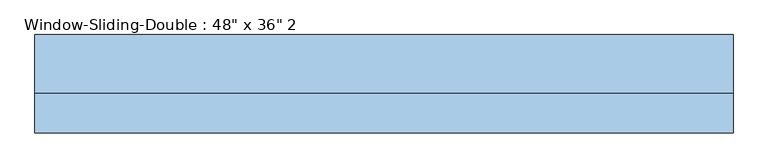
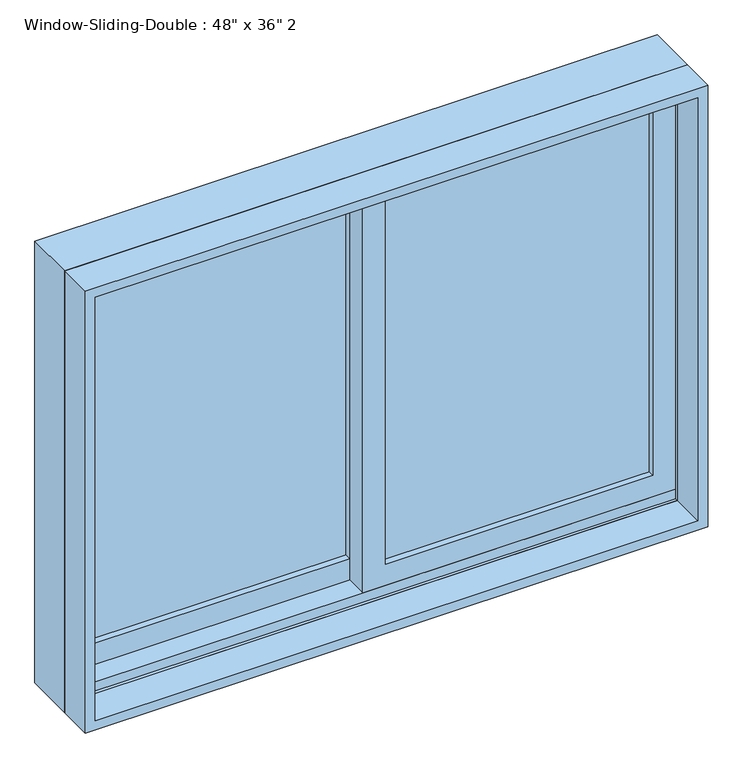
"""IFC4 building model written with IfcOpenShell, lengths in millimetres: window geometry."""

from ifc_helpers import new_model, si_unit, frame, origin, place, context, project, spatial, polyline, outline, extrude, faceted_brep, source, transform, mapped, element, save


def window_547996ef(model_context):
    return source(origin(), model_context, "Body", "SolidModel", [
        faceted_brep([(-609.6, -10.16, 914.4), (-609.6, 91.44, 914.4), (609.6, 91.44, 914.4), (609.6, -10.16, 914.4), (-568.6778905, 91.44, 1787.8778905), (-568.6778905, 85.09, 1787.8778905), (-568.6778905, 85.09, 933.45), (-568.6778905, 91.44, 933.45), (568.6778905, 85.09, 1787.8778905), (568.6778905, 85.09, 933.45), (590.55, 85.09, 933.45), (590.55, 85.09, 1809.75), (-590.55, 85.09, 1809.75), (-590.55, 85.09, 933.45), (-590.55, -10.16, 1809.75), (-590.55, -10.16, 933.45), (-590.55, -3.81, 933.45), (-590.55, -3.81, 952.5), (-590.55, 40.64, 952.5), (-590.55, 40.64, 933.45), (609.6, -10.16, 1828.8), (-609.6, -10.16, 1828.8), (590.55, -10.16, 1809.75), (590.55, -10.16, 933.45), (-609.6, 91.44, 1828.8), (609.6, 91.44, 1828.8), (568.6778905, 91.44, 933.45), (568.6778905, 91.44, 1787.8778905), (590.55, 40.64, 933.45), (590.55, 40.64, 952.5), (590.55, -3.81, 952.5), (590.55, -3.81, 933.45)], [[[0, 1, 2, 3]], [[4, 5, 6, 7]], [[5, 8, 9, 10, 11, 12, 13, 6]], [[12, 14, 15, 16, 17, 18, 19, 13]], [[0, 3, 20, 21], [22, 23, 15, 14]], [[24, 1, 0, 21]], [[2, 1, 24, 25], [4, 7, 26, 27]], [[5, 4, 27, 8]], [[12, 11, 22, 14]], [[21, 20, 25, 24]], [[8, 27, 26, 9]], [[22, 11, 10, 28, 29, 30, 31, 23]], [[20, 3, 2, 25]], [[26, 7, 6, 13, 19, 28, 10, 9]], [[28, 19, 18, 29]], [[29, 18, 17, 30]], [[30, 17, 16, 31]], [[15, 23, 31, 16]]]),
        extrude(outline(polyline([(1828.8, -609.6), (914.4, -609.6), (914.4, 609.6), (1828.8, 609.6), (1828.8, -609.6)]), holes=[polyline([(1809.75, 590.55), (933.45, 590.55), (933.45, -590.55), (1809.75, -590.55), (1809.75, 590.55)])]), frame((0.0, -80.01, 0.0), z_axis=(0.0, 1.0, 0.0), x_axis=(0.0, 0.0, 1.0)), (0.0, 0.0, 1.0), 69.85),
        extrude(outline(polyline([(546.1, 27.94), (546.1, 21.59), (22.225, 21.59), (22.225, 27.94), (546.1, 27.94)])), frame((0.0, 0.0, 996.95), z_axis=(0.0, 0.0, 1.0), x_axis=(1.0, 0.0, 0.0)), (0.0, 0.0, 1.0), 768.35),
        extrude(outline(polyline([(546.1, 15.24), (546.1, 8.89), (22.225, 8.89), (22.225, 15.24), (546.1, 15.24)])), frame((0.0, 0.0, 996.95), z_axis=(0.0, 0.0, 1.0), x_axis=(1.0, 0.0, 0.0)), (0.0, 0.0, 1.0), 768.35),
        extrude(outline(polyline([(-22.225, 72.39), (-22.225, 66.04), (-546.1, 66.04), (-546.1, 72.39), (-22.225, 72.39)])), frame((0.0, 0.0, 996.95), z_axis=(0.0, 0.0, 1.0), x_axis=(1.0, 0.0, 0.0)), (0.0, 0.0, 1.0), 768.35),
        extrude(outline(polyline([(-22.225, 59.69), (-22.225, 53.34), (-546.1, 53.34), (-546.1, 59.69), (-22.225, 59.69)])), frame((0.0, 0.0, 996.95), z_axis=(0.0, 0.0, 1.0), x_axis=(1.0, 0.0, 0.0)), (0.0, 0.0, 1.0), 768.35),
        extrude(outline(polyline([(933.45, -590.55), (933.45, 22.225), (1809.75, 22.225), (1809.75, -590.55), (933.45, -590.55)]), holes=[polyline([(1765.3, -22.225), (996.95, -22.225), (996.95, -546.1), (1765.3, -546.1), (1765.3, -22.225)])]), frame((0.0, 40.64, 0.0), z_axis=(0.0, 1.0, 0.0), x_axis=(0.0, 0.0, 1.0)), (0.0, 0.0, 1.0), 44.45),
        extrude(outline(polyline([(952.5, 590.55), (1809.75, 590.55), (1809.75, -22.225), (952.5, -22.225), (952.5, 590.55)]), holes=[polyline([(996.95, 22.225), (1765.3, 22.225), (1765.3, 546.1), (996.95, 546.1), (996.95, 22.225)])]), frame((0.0, -3.81, 0.0), z_axis=(0.0, 1.0, 0.0), x_axis=(0.0, 0.0, 1.0)), (0.0, 0.0, 1.0), 44.45),
    ])


if __name__ == "__main__":
    model = new_model("IFC4")
    model_context = context("Model", 3, world=origin())
    ifc_project = project(units=[si_unit("LENGTHUNIT", "METRE", prefix="MILLI")], contexts=[model_context])
    site = spatial("IfcSite", under=ifc_project)
    building = spatial("IfcBuilding", under=site)
    placement = place(None, origin())
    window_shape = window_547996ef(model_context)
    element("IfcWindow", 1, ObjectType="Window-Sliding-Double : 48\" x 36\" 2", at=placement, inside=building, context=model_context, shape_type="MappedRepresentation", body=[
        mapped(window_shape, transform((0.0, 0.0, 0.0), x_axis=(1.0, 0.0, 0.0), y_axis=(0.0, 1.0, 0.0), z_axis=(0.0, 0.0, 1.0))),
    ])
    save(model, "model.ifc")

# Revit data of these elements
# Type "Window-Sliding-Double : 48\" x 36\" 2"
#   Type Mark = "16"
#   Fire Rating = "0.5h"
#   Assembly Code = "B2020100"
#   Analytic Construction = "Double glazing - domestic"
#   Window Inset [instance default] = 0' - 0"
#   Wall Thickness [instance default] = 0' - 6"
#   Visual Light Transmittance = 0.81
#   Thermal Resistance (R) = 0.319569 (m²·K)/W
#   Solar Heat Gain Coefficient = 0.76
#   Muntin Width = 1' - 8 5/8"
#   Muntin Height = 2' - 6 1/4"
#   Interior Wall Closure [instance default] = 0' - 2 3/4"
#   Heat Transfer Coefficient (U) = 3.12929 W/(m²·K)
#   Frame Extension [instance default] = 0' - 0 1/4"
#   Exterior Wall Closure [instance default] = 0' - 1 1/4"
#   Rough Width = 4' - 0 1/2"
#   Rough Height = 3' - 0 1/2"
#   Height = 3' - 0"
#   Extension Jamb [instance default] = 0' - 2 3/4"
#   Default Sill Height = 3' - 0"
#   Width = 4' - 0"
#   Interior Trim Visibility [instance default] = yes
#   Indicator Visibility [instance default] = yes
#   Exterior Trim Visibility [instance default] = yes
#   Muntin Visibility = no
#   Extension Jamb Visibility [instance default] = yes
#   Muntin Pattern = Muntin Pattern_2x2 : Muntin Pattern_2x2
#   Interior Trim Material = Wood - Stained
#   Interior Trim = Trim-Window-Interior-Flat : Picture Frame
#   Interior Frame Material = Wood - Stained
#   Glass Panel Material = Glass
#   Exterior Trim Material = Clad - White
#   Exterior Trim = Trim-Window-Exterior-Flat : with Sill
#   Exterior Frame Material = Clad - White
#   Wall Closure = (empty or 0)
# Element 1 (IfcWindow, "Window-Sliding-Double : 48\" x 36\" 2")
#   Materials on its faces: "Wood - Stained", "Glass", "Clad - White"
# Materials
#   "Wood - Stained": class "Wood", colour RGB 224 178 126, transparency 0, Cost = 0
#   "Glass": class "Glass", colour RGB 218 227 224, transparency 0.85, Description = "Soda Lime Glass", Cost = 0
#   "Clad - White": class "Wood", colour RGB 242 242 238, transparency 0, Cost = 0
